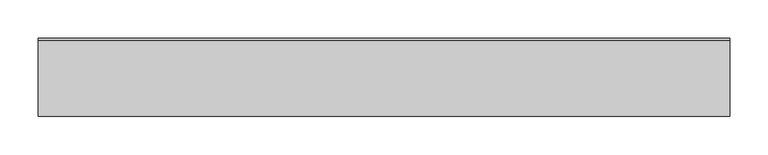
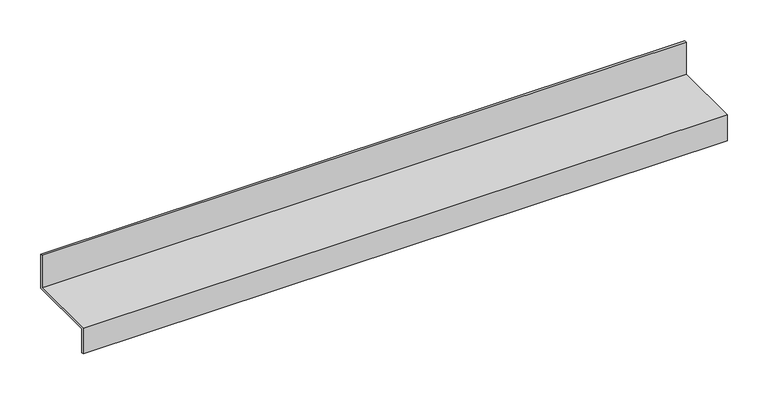
"""IFC4 building model written with IfcOpenShell, lengths in millimetres: proxy geometry, Generic Models 7:Generic Models 1:8:Generic Models 1:8 : Generic Models 7:Generic Models 1:337419:19 : Generic Models 7:Generic Models 1:8:Generic Models 1:8 : Generic Models 7:Generic Models 1:337419:315935."""

from ifc_helpers import new_model, si_unit, frame, origin, place, context, project, spatial, polyline, outline, extrude, source, transform, mapped, element, save


def generic_models_e3d6314e(model_context):
    return source(origin(), model_context, "Body", "SweptSolid", [
        extrude(outline(polyline([(-579121.2152286, 3717.925), (-579121.2152286, 3682.603125), (-579123.9933536, 3682.603125), (-579123.9933536, 3720.703125), (-579024.1070091, 3720.703125), (-579024.1070091, 3768.725), (-579021.3288841, 3768.725), (-579021.3288841, 3717.925), (-579121.2152286, 3717.925)])), frame((569545.1440816, 0.0, 0.0), z_axis=(1.0, 0.0, 0.0), x_axis=(0.0, 1.0, 0.0)), (0.0, 0.0, 1.0), 907.4926423),
    ])


if __name__ == "__main__":
    model = new_model("IFC4")
    model_context = context("Model", 3, world=origin())
    ifc_project = project(units=[si_unit("LENGTHUNIT", "METRE", prefix="MILLI")], contexts=[model_context])
    site = spatial("IfcSite", under=ifc_project)
    building = spatial("IfcBuilding", under=site)
    placement = place(None, origin())
    generic_models_shape = generic_models_e3d6314e(model_context)
    element("IfcBuildingElementProxy", 1, Name="Generic Models 7:Generic Models 1:8:Generic Models 1:8 : Generic Models 7:Generic Models 1:337419:19 : Generic Models 7:Generic Models 1:8:Generic Models 1:8 : Generic Models 7:Generic Models 1:337419:315935", ObjectType="Generic Models 7:Generic Models 1:8:Generic Models 1:8 : Generic Models 7:Generic Models 1:337419:19 : Generic Models 7:Generic Models 1:8:Generic Models 1:8 : Generic Models 7:Generic Models 1:337419:315935", at=placement, inside=building, context=model_context, shape_type="MappedRepresentation", body=[
        mapped(generic_models_shape, transform((0.0, 0.0, 0.0), x_axis=(1.0, 0.0, 0.0), y_axis=(0.0, 1.0, 0.0), z_axis=(0.0, 0.0, 1.0))),
    ])
    save(model, "model.ifc")

# Revit data of these elements
# Type "Generic Models 7:Generic Models 1:8:Generic Models 1:8 : Generic Models 7:Generic Models 1:337419:19 : Generic Models 7:Generic Models 1:8:Generic Models 1:8 : Generic Models 7:Generic Models 1:337419:315935"
#   NameOverride = "Generic Models 7:Generic Models 1:8:Generic Models 1:8 : Generic Models 7:Generic Models 1:337419:315935"
#   ObjectTypeOverride = "Generic Models 1:8 : Generic Models 7:Generic Models 1:337419"
#   Reference = "Generic Models 1"
#   Tag = "315935"
# Element 1 (IfcBuildingElementProxy, "Generic Models 7:Generic Models 1:8:Generic Models 1:8 : Generic Models 7:Generic Models 1:337419:19 : Generic Models 7:Generic Models 1:8:Generic Models 1:8 : Generic Models 7:Generic Models 1:337419:315935")
#   Materials on its faces: "11 GA. ALUM. BRAKE METAL (ALIGN WITH B.M. @ STOREFRONT/RESIN/POLYCARBONATE)"
# Materials
#   "11 GA. ALUM. BRAKE METAL (ALIGN WITH B.M. @ STOREFRONT/RESIN/POLYCARBONATE)": class "Unassigned", colour RGB 210 209 208, transparency 0, Cost = 0
